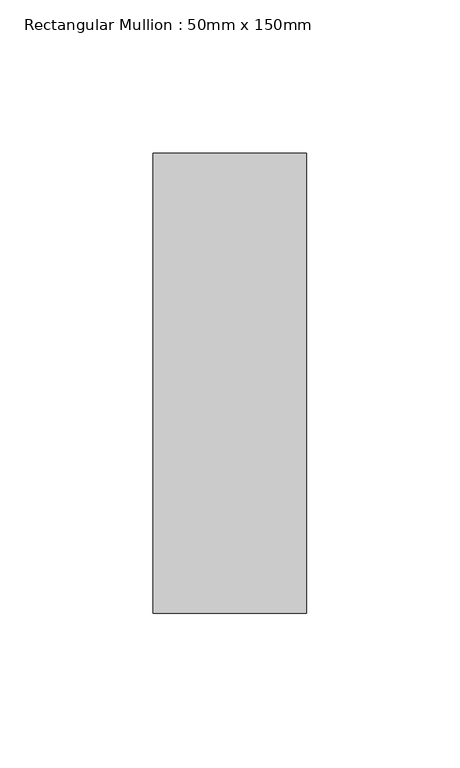
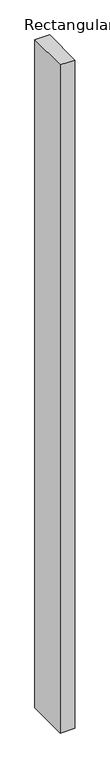
"""IFC4 building model written with IfcOpenShell, lengths in millimetres: member geometry, Rectangular Mullion : 50mm x 150mm."""

import ifcopenshell
import ifcopenshell.guid

model = None  # the IFC model being written
_history = None  # IfcOwnerHistory: only IFC2X3 demands one
_inside = {}  # id of a spatial element -> (the spatial element, [elements in it])
_under = {}  # id of a project, library or spatial element -> (it, [spatial elements below it])
_declared = {}  # id of a project -> (the project, [libraries it declares])
_typed = {}  # id of a type object -> (the type object, [elements of that type])
_made_of = {}  # id of a material, layer set ... -> (it, [elements and type objects made of it])


def new_model(schema):
    """Start an empty IFC model of exactly this schema.

    Asked for "IFC4X3", IfcOpenShell would pick the latest addendum, in which some entities
    have other attributes; the version numbers below select the first issue.
    IFC2X3 requires an IfcOwnerHistory on every rooted entity: one is made here for all.
    """
    global model, _history
    if schema == "IFC4X3":
        model = ifcopenshell.file(schema_version=(4, 3, 0, 0))
    else:
        model = ifcopenshell.file(schema=schema)
    _inside.clear()
    _under.clear()
    _declared.clear()
    _typed.clear()
    _made_of.clear()
    _history = None
    if model.schema == "IFC2X3":
        org = make("IfcOrganization", Name="unknown")
        user = make(
            "IfcPersonAndOrganization",
            ThePerson=make("IfcPerson", FamilyName="unknown"),
            TheOrganization=org,
        )
        app = make(
            "IfcApplication",
            ApplicationDeveloper=org,
            Version="unknown",
            ApplicationFullName="unknown",
            ApplicationIdentifier="unknown",
        )
        _history = make(
            "IfcOwnerHistory",
            OwningUser=user,
            OwningApplication=app,
            ChangeAction="ADDED",
            CreationDate=0,
        )
    return model


def make(cls, **values):
    """One entity of the class cls with the attributes given. An attribute that is None is left unset."""
    return model.create_entity(
        cls, **{name: value for name, value in values.items() if value is not None}
    )


def rooted(cls, **values):
    """An entity with a GlobalId (a new one), such as an element, a storey or a relation."""
    return make(cls, GlobalId=ifcopenshell.guid.new(), OwnerHistory=_history, **values)


def si_unit(unit_type, name, prefix=None):
    """IfcSIUnit, for example si_unit("LENGTHUNIT", "METRE", prefix="MILLI")."""
    return make("IfcSIUnit", UnitType=unit_type, Prefix=prefix, Name=name)


def assignment(units):
    """IfcUnitAssignment: the units of a project."""
    return None if units is None else make("IfcUnitAssignment", Units=units)


def point(xyz):
    """IfcCartesianPoint."""
    return None if xyz is None else make("IfcCartesianPoint", Coordinates=xyz)


def direction(xyz):
    """IfcDirection."""
    return None if xyz is None else make("IfcDirection", DirectionRatios=xyz)


def frame(location, z_axis=None, x_axis=None):
    """IfcAxis2Placement3D, a coordinate frame: its origin and axes. An axis left out is left unset."""
    return make(
        "IfcAxis2Placement3D",
        Location=point(location),
        Axis=direction(z_axis),
        RefDirection=direction(x_axis),
    )


def origin():
    """The frame at (0, 0, 0) with its axes left unset."""
    return frame((0.0, 0.0, 0.0))


def place(relative_to, where):
    """IfcLocalPlacement: puts the frame where relative to a parent placement (None: the world)."""
    return make(
        "IfcLocalPlacement", PlacementRelTo=relative_to, RelativePlacement=where
    )


def context(
    kind, dimensions, precision=None, world=None, true_north=None, identifier=None
):
    """IfcGeometricRepresentationContext, for example the 3D "Model" context."""
    return make(
        "IfcGeometricRepresentationContext",
        ContextIdentifier=identifier,
        ContextType=kind,
        CoordinateSpaceDimension=dimensions,
        Precision=precision,
        WorldCoordinateSystem=world,
        TrueNorth=true_north,
    )


def project(units=None, contexts=None):
    """IfcProject with its units and contexts."""
    return rooted(
        "IfcProject",
        Name="project",
        RepresentationContexts=contexts,
        UnitsInContext=assignment(units),
    )


def spatial(cls, under=None, at=None, **own):
    """A site, building, storey or space (cls), placed at a placement, below another one or the project."""
    s = rooted(cls, ObjectPlacement=at, **own)
    if under is not None:
        _under.setdefault(under.id(), (under, []))[1].append(s)
    return s


def polyline(points):
    """IfcPolyline through the points."""
    return make("IfcPolyline", Points=[point(p) for p in points])


def outline(outer, holes=None, kind="AREA"):
    """IfcArbitraryClosedProfileDef: a profile drawn as a closed curve; with holes, ...WithVoids."""
    if holes is None:
        return make("IfcArbitraryClosedProfileDef", ProfileType=kind, OuterCurve=outer)
    return make(
        "IfcArbitraryProfileDefWithVoids",
        ProfileType=kind,
        OuterCurve=outer,
        InnerCurves=holes,
    )


def extrude(swept, where, along, depth):
    """IfcExtrudedAreaSolid: the profile swept, set in the frame where, extruded along a direction by depth."""
    return make(
        "IfcExtrudedAreaSolid",
        SweptArea=swept,
        Position=where,
        ExtrudedDirection=direction(along),
        Depth=depth,
    )


def shape(context_of_items, identifier, shape_type, items):
    """IfcShapeRepresentation: the items that make up one representation, for example the "Body"."""
    return make(
        "IfcShapeRepresentation",
        ContextOfItems=context_of_items,
        RepresentationIdentifier=identifier,
        RepresentationType=shape_type,
        Items=items,
    )


def source(mapping_origin, context_of_items, identifier, shape_type, items):
    """IfcRepresentationMap: a shape defined once, which mapped items show again and again."""
    return make(
        "IfcRepresentationMap",
        MappingOrigin=mapping_origin,
        MappedRepresentation=shape(context_of_items, identifier, shape_type, items),
    )


def transform(
    local_origin,
    x_axis=None,
    y_axis=None,
    z_axis=None,
    scale=None,
    scale2=None,
    scale3=None,
    uniform=True,
):
    """IfcCartesianTransformationOperator3D, or its non-uniform kind. x_axis, y_axis, z_axis: its Axis1, 2, 3."""
    if uniform:
        return make(
            "IfcCartesianTransformationOperator3D",
            Axis1=direction(x_axis),
            Axis2=direction(y_axis),
            LocalOrigin=point(local_origin),
            Scale=scale,
            Axis3=direction(z_axis),
        )
    return make(
        "IfcCartesianTransformationOperator3DnonUniform",
        Axis1=direction(x_axis),
        Axis2=direction(y_axis),
        LocalOrigin=point(local_origin),
        Scale=scale,
        Axis3=direction(z_axis),
        Scale2=scale2,
        Scale3=scale3,
    )


def mapped(mapping_source, mapping_target):
    """IfcMappedItem: shows the shape of a source again, moved by a transform."""
    return make(
        "IfcMappedItem", MappingSource=mapping_source, MappingTarget=mapping_target
    )


def made_of(thing, what):
    """Note that an element or type object is made of a material, layer set ...; save() writes the relation."""
    if what is not None:
        _made_of.setdefault(what.id(), (what, []))[1].append(thing)
    return thing


def element(
    cls,
    number,
    at=None,
    inside=None,
    cuts=None,
    type_object=None,
    material=None,
    context=None,
    identifier="Body",
    shape_type=None,
    held_by="IfcProductDefinitionShape",
    body=None,
    shapes=None,
    **own,
):
    """One element of the class cls, such as IfcWall. Its Tag is "e" and its number.

    at: its placement. inside: the storey or other place that contains it. cuts: it is an
    opening in that element (IfcRelVoidsElement). A single representation is given by context,
    identifier, shape_type and body (its items); several are given by shapes. held_by: the class
    of the entity that holds the representations. save() writes the other relations.
    """
    e = rooted(cls, Tag="e%d" % number, ObjectPlacement=at, **own)
    if body is not None:
        shapes = [shape(context, identifier, shape_type, body)]
    if shapes is not None:
        e.Representation = make(held_by, Representations=shapes)
    if inside is not None:
        _inside.setdefault(inside.id(), (inside, []))[1].append(e)
    if cuts is not None:
        rooted(
            "IfcRelVoidsElement", RelatingBuildingElement=cuts, RelatedOpeningElement=e
        )
    if type_object is not None:
        _typed.setdefault(type_object.id(), (type_object, []))[1].append(e)
    return made_of(e, material)


def aggregate(whole, parts):
    """IfcRelAggregates: a whole, such as a stair, and the parts it consists of."""
    return rooted("IfcRelAggregates", RelatingObject=whole, RelatedObjects=parts)


def save(model, path):
    """Write the relations noted so far, then the file.

    IfcRelAggregates (storeys below a building ...), IfcRelContainedInSpatialStructure (elements
    in a storey), IfcRelDefinesByType, IfcRelAssociatesMaterial and IfcRelDeclares: one each for
    every whole, place, type object, material and project.
    """
    for whole, parts in _under.values():
        aggregate(whole, parts)
    for where, things in _inside.values():
        rooted(
            "IfcRelContainedInSpatialStructure",
            RelatedElements=things,
            RelatingStructure=where,
        )
    for kind, things in _typed.values():
        rooted("IfcRelDefinesByType", RelatedObjects=things, RelatingType=kind)
    for what, things in _made_of.values():
        rooted("IfcRelAssociatesMaterial", RelatedObjects=things, RelatingMaterial=what)
    for by, libraries in _declared.values():
        rooted("IfcRelDeclares", RelatingContext=by, RelatedDefinitions=libraries)
    model.write(path)


def rectangular_mullion_50mm_x_150mm_f904506f(model_context):
    return source(origin(), model_context, "Body", "SweptSolid", [
        extrude(outline(polyline([(25.0, 75.0), (25.0, -75.0), (-25.0, -75.0), (-25.0, 75.0), (25.0, 75.0)])), frame((0.0, 0.0, -2420.0), z_axis=(0.0, 0.0, 1.0), x_axis=(1.0, 0.0, 0.0)), (0.0, 0.0, 1.0), 2420.0),
    ])


if __name__ == "__main__":
    model = new_model("IFC4")
    model_context = context("Model", 3, world=origin())
    ifc_project = project(units=[si_unit("LENGTHUNIT", "METRE", prefix="MILLI")], contexts=[model_context])
    site = spatial("IfcSite", under=ifc_project)
    building = spatial("IfcBuilding", under=site)
    placement = place(None, origin())
    rectangular_mullion_50mm_x_150mm_shape = rectangular_mullion_50mm_x_150mm_f904506f(model_context)
    element("IfcMember", 1, ObjectType="Rectangular Mullion : 50mm x 150mm", at=placement, inside=building, context=model_context, shape_type="MappedRepresentation", body=[
        mapped(rectangular_mullion_50mm_x_150mm_shape, transform((0.0, 0.0, 0.0), x_axis=(1.0, 0.0, 0.0), y_axis=(0.0, 1.0, 0.0), z_axis=(0.0, 0.0, 1.0))),
    ])
    save(model, "model.ifc")

# Revit data of these elements
# Type "Rectangular Mullion : 50mm x 150mm"
#   built-in parameter 1007304 = 0.492126 (stored number, unit not read)
#   built-in parameter 1007301 = 0.082021 (stored number, unit not read)
#   built-in parameter 1007300 = 0.082021 (stored number, unit not read)
# Element 1 (IfcMember, "Rectangular Mullion : 50mm x 150mm")
#   Materials on its faces: "Aluminum"
# Materials
#   "Aluminum": class "Metal", colour RGB 244 244 244, transparency 0, Description = "Aluminum 6061", Cost = 0
